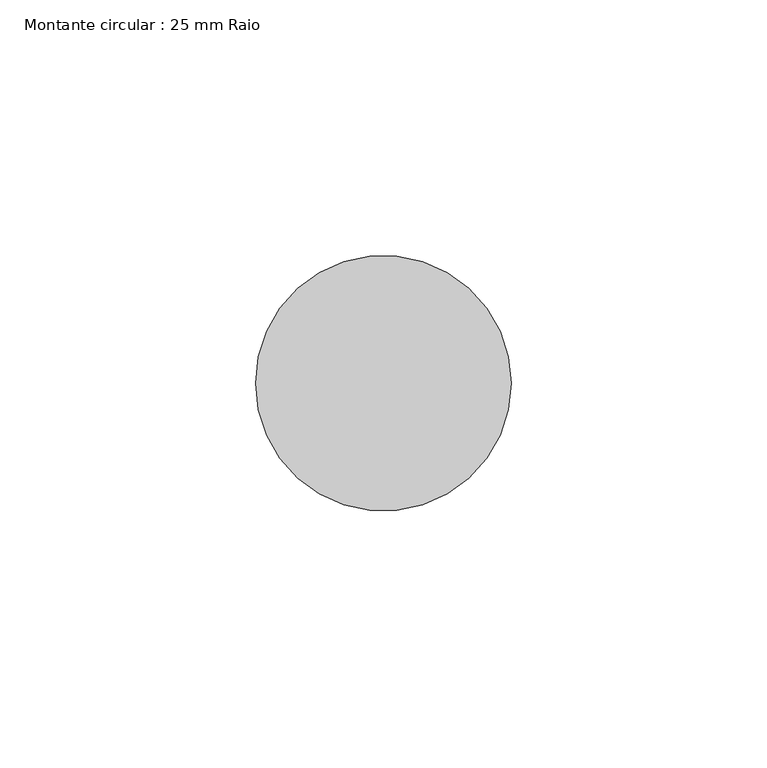
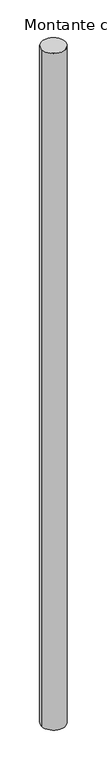
"""IFC4 building model written with IfcOpenShell, lengths in millimetres: member geometry, Montante circular : 25 mm Raio."""

from ifc_helpers import new_model, si_unit, point, frame, origin, origin_2d, place, context, project, spatial, circle_curve, trimmed, segment, composite_curve, outline, extrude, source, transform, mapped, element, save


def montante_circular_25_mm_raio_d4c4f207(model_context):
    return source(origin(), model_context, "Body", "SweptSolid", [
        extrude(outline(composite_curve([segment(trimmed(circle_curve(origin_2d(), 25.0), [point((25.0, 0.0))], [point((-25.0, 0.0))], False, "CARTESIAN"), True, "CONTINUOUS"), segment(trimmed(circle_curve(origin_2d(), 25.0), [point((-25.0, 0.0))], [point((25.0, 0.0))], False, "CARTESIAN"), True, "CONTINUOUS")], self_intersect=False)), frame((0.0, 0.0, -1506.2958402), z_axis=(0.0, 0.0, 1.0), x_axis=(1.0, 0.0, 0.0)), (0.0, 0.0, 1.0), 1506.2958402),
    ])


if __name__ == "__main__":
    model = new_model("IFC4")
    model_context = context("Model", 3, world=origin())
    ifc_project = project(units=[si_unit("LENGTHUNIT", "METRE", prefix="MILLI")], contexts=[model_context])
    site = spatial("IfcSite", under=ifc_project)
    building = spatial("IfcBuilding", under=site)
    placement = place(None, origin())
    montante_circular_25_mm_raio_shape = montante_circular_25_mm_raio_d4c4f207(model_context)
    element("IfcMember", 1, ObjectType="Montante circular : 25 mm Raio", at=placement, inside=building, context=model_context, shape_type="MappedRepresentation", body=[
        mapped(montante_circular_25_mm_raio_shape, transform((0.0, 0.0, 0.0), x_axis=(1.0, 0.0, 0.0), y_axis=(0.0, 1.0, 0.0), z_axis=(0.0, 0.0, 1.0))),
    ])
    save(model, "model.ifc")

# Revit data of these elements
# Type "Montante circular : 25 mm Raio"
#   built-in parameter 1007350 = 0.082021 (stored number, unit not read)
# Element 1 (IfcMember, "Montante circular : 25 mm Raio")
#   Materials on its faces: "Alumín."
# Materials
#   "Alumín.": class "Metal", colour RGB 247 247 247, transparency 0, Description = "Alumín. 6061", Cost = 0
